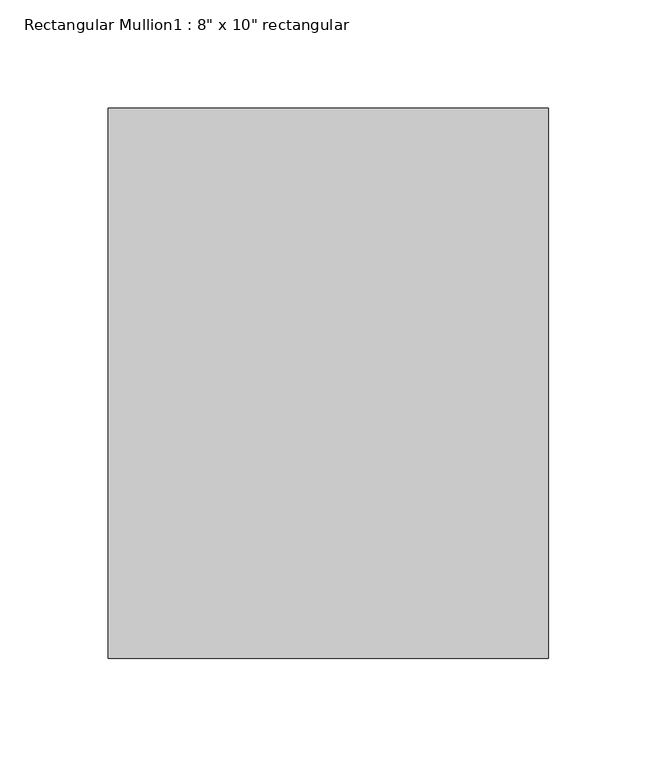
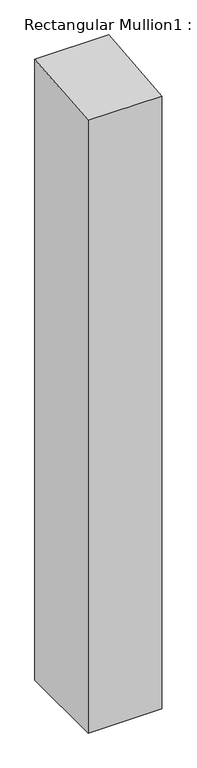
"""IFC4 building model written with IfcOpenShell, lengths in millimetres: member geometry."""

from ifc_helpers import new_model, si_unit, frame, origin, place, context, project, spatial, polyline, outline, extrude, source, transform, mapped, element, save


def member_84ccbaea(model_context):
    return source(origin(), model_context, "Body", "SweptSolid", [
        extrude(outline(polyline([(-127.0, -11.9934772), (127.0, 11.9934772), (127.0, -1797.05), (-127.0, -1797.05), (-127.0, -11.9934772)])), frame((-101.6, 0.0, 0.0), z_axis=(1.0, 0.0, 0.0), x_axis=(0.0, 1.0, 0.0)), (0.0, 0.0, 1.0), 203.2),
    ])


if __name__ == "__main__":
    model = new_model("IFC4")
    model_context = context("Model", 3, world=origin())
    ifc_project = project(units=[si_unit("LENGTHUNIT", "METRE", prefix="MILLI")], contexts=[model_context])
    site = spatial("IfcSite", under=ifc_project)
    building = spatial("IfcBuilding", under=site)
    placement = place(None, origin())
    member_shape = member_84ccbaea(model_context)
    element("IfcMember", 1, ObjectType="Rectangular Mullion1 : 8\" x 10\" rectangular", at=placement, inside=building, context=model_context, shape_type="MappedRepresentation", body=[
        mapped(member_shape, transform((0.0, 0.0, 0.0), x_axis=(1.0, 0.0, 0.0), y_axis=(0.0, 1.0, 0.0), z_axis=(0.0, 0.0, 1.0))),
    ])
    save(model, "model.ifc")

# Revit data of these elements
# Type "Rectangular Mullion1 : 8\" x 10\" rectangular"
#   built-in parameter 1007304 = 0.833333 (stored number, unit not read)
#   built-in parameter 1007301 = 0.333333 (stored number, unit not read)
#   built-in parameter 1007300 = 0.333333 (stored number, unit not read)
# Element 1 (IfcMember, "Rectangular Mullion1 : 8\" x 10\" rectangular")
#   Materials on its faces: "support-frame"
# Materials
#   "support-frame": class "Unassigned", colour RGB 233 233 233, transparency 0, Cost = 0
